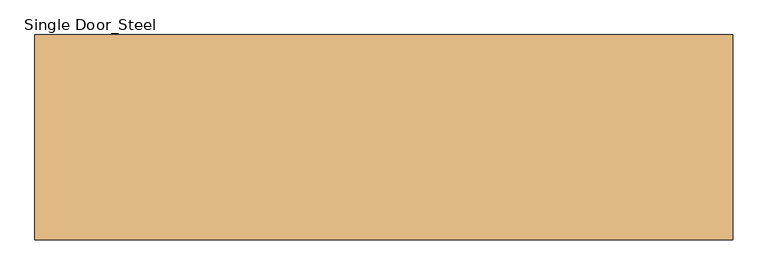
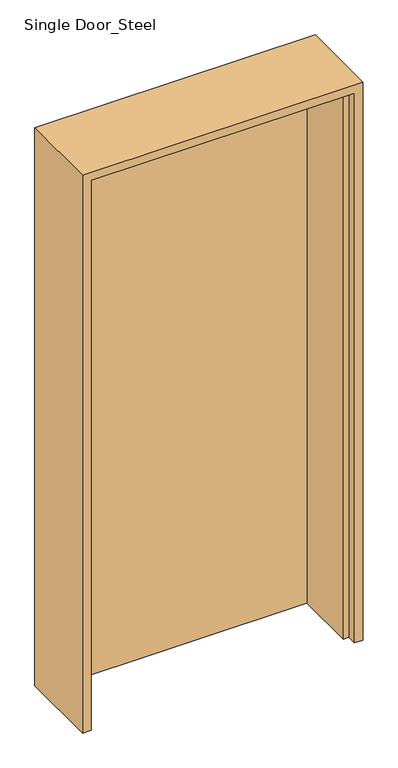
"""IFC4 building model written with IfcOpenShell, lengths in millimetres: door geometry, Single Door_Steel : H_DR_AR_B12_Single Door_Steel_W1000xH2100."""

import ifcopenshell
import ifcopenshell.guid

model = None  # the IFC model being written
_history = None  # IfcOwnerHistory: only IFC2X3 demands one
_inside = {}  # id of a spatial element -> (the spatial element, [elements in it])
_under = {}  # id of a project, library or spatial element -> (it, [spatial elements below it])
_declared = {}  # id of a project -> (the project, [libraries it declares])
_typed = {}  # id of a type object -> (the type object, [elements of that type])
_made_of = {}  # id of a material, layer set ... -> (it, [elements and type objects made of it])


def new_model(schema):
    """Start an empty IFC model of exactly this schema.

    Asked for "IFC4X3", IfcOpenShell would pick the latest addendum, in which some entities
    have other attributes; the version numbers below select the first issue.
    IFC2X3 requires an IfcOwnerHistory on every rooted entity: one is made here for all.
    """
    global model, _history
    if schema == "IFC4X3":
        model = ifcopenshell.file(schema_version=(4, 3, 0, 0))
    else:
        model = ifcopenshell.file(schema=schema)
    _inside.clear()
    _under.clear()
    _declared.clear()
    _typed.clear()
    _made_of.clear()
    _history = None
    if model.schema == "IFC2X3":
        org = make("IfcOrganization", Name="unknown")
        user = make(
            "IfcPersonAndOrganization",
            ThePerson=make("IfcPerson", FamilyName="unknown"),
            TheOrganization=org,
        )
        app = make(
            "IfcApplication",
            ApplicationDeveloper=org,
            Version="unknown",
            ApplicationFullName="unknown",
            ApplicationIdentifier="unknown",
        )
        _history = make(
            "IfcOwnerHistory",
            OwningUser=user,
            OwningApplication=app,
            ChangeAction="ADDED",
            CreationDate=0,
        )
    return model


def make(cls, **values):
    """One entity of the class cls with the attributes given. An attribute that is None is left unset."""
    return model.create_entity(
        cls, **{name: value for name, value in values.items() if value is not None}
    )


def rooted(cls, **values):
    """An entity with a GlobalId (a new one), such as an element, a storey or a relation."""
    return make(cls, GlobalId=ifcopenshell.guid.new(), OwnerHistory=_history, **values)


def si_unit(unit_type, name, prefix=None):
    """IfcSIUnit, for example si_unit("LENGTHUNIT", "METRE", prefix="MILLI")."""
    return make("IfcSIUnit", UnitType=unit_type, Prefix=prefix, Name=name)


def assignment(units):
    """IfcUnitAssignment: the units of a project."""
    return None if units is None else make("IfcUnitAssignment", Units=units)


def point(xyz):
    """IfcCartesianPoint."""
    return None if xyz is None else make("IfcCartesianPoint", Coordinates=xyz)


def direction(xyz):
    """IfcDirection."""
    return None if xyz is None else make("IfcDirection", DirectionRatios=xyz)


def frame(location, z_axis=None, x_axis=None):
    """IfcAxis2Placement3D, a coordinate frame: its origin and axes. An axis left out is left unset."""
    return make(
        "IfcAxis2Placement3D",
        Location=point(location),
        Axis=direction(z_axis),
        RefDirection=direction(x_axis),
    )


def origin():
    """The frame at (0, 0, 0) with its axes left unset."""
    return frame((0.0, 0.0, 0.0))


def origin_with_axes():
    """The frame at (0, 0, 0) with the z axis (0, 0, 1) and the x axis (1, 0, 0) written out."""
    return frame((0.0, 0.0, 0.0), z_axis=(0.0, 0.0, 1.0), x_axis=(1.0, 0.0, 0.0))


def place(relative_to, where):
    """IfcLocalPlacement: puts the frame where relative to a parent placement (None: the world)."""
    return make(
        "IfcLocalPlacement", PlacementRelTo=relative_to, RelativePlacement=where
    )


def context(
    kind, dimensions, precision=None, world=None, true_north=None, identifier=None
):
    """IfcGeometricRepresentationContext, for example the 3D "Model" context."""
    return make(
        "IfcGeometricRepresentationContext",
        ContextIdentifier=identifier,
        ContextType=kind,
        CoordinateSpaceDimension=dimensions,
        Precision=precision,
        WorldCoordinateSystem=world,
        TrueNorth=true_north,
    )


def project(units=None, contexts=None):
    """IfcProject with its units and contexts."""
    return rooted(
        "IfcProject",
        Name="project",
        RepresentationContexts=contexts,
        UnitsInContext=assignment(units),
    )


def spatial(cls, under=None, at=None, **own):
    """A site, building, storey or space (cls), placed at a placement, below another one or the project."""
    s = rooted(cls, ObjectPlacement=at, **own)
    if under is not None:
        _under.setdefault(under.id(), (under, []))[1].append(s)
    return s


def polyline(points):
    """IfcPolyline through the points."""
    return make("IfcPolyline", Points=[point(p) for p in points])


def outline(outer, holes=None, kind="AREA"):
    """IfcArbitraryClosedProfileDef: a profile drawn as a closed curve; with holes, ...WithVoids."""
    if holes is None:
        return make("IfcArbitraryClosedProfileDef", ProfileType=kind, OuterCurve=outer)
    return make(
        "IfcArbitraryProfileDefWithVoids",
        ProfileType=kind,
        OuterCurve=outer,
        InnerCurves=holes,
    )


def extrude(swept, where, along, depth):
    """IfcExtrudedAreaSolid: the profile swept, set in the frame where, extruded along a direction by depth."""
    return make(
        "IfcExtrudedAreaSolid",
        SweptArea=swept,
        Position=where,
        ExtrudedDirection=direction(along),
        Depth=depth,
    )


def faces_of(points, faces, orient=None, outer=None):
    """IfcFace entities. A face is a list of loops; a loop is a list of indices into points, from 0.

    orient and outer hold one flag for each loop. By default every Orientation is true, the
    first loop of a face is its IfcFaceOuterBound and the others are IfcFaceBound.
    """
    made = []
    for i, loops in enumerate(faces):
        bounds = []
        for j, loop in enumerate(loops):
            is_outer = j == 0 if outer is None else outer[i][j]
            bounds.append(
                make(
                    "IfcFaceOuterBound" if is_outer else "IfcFaceBound",
                    Bound=make("IfcPolyLoop", Polygon=[points[k] for k in loop]),
                    Orientation=True if orient is None else orient[i][j],
                )
            )
        made.append(make("IfcFace", Bounds=bounds))
    return made


def faceted_brep(points, faces, orient=None, outer=None, voids=None):
    """IfcFacetedBrep: a solid bounded by flat faces; with voids (closed shells), ...WithVoids."""
    shared = [point(p) for p in points]
    hull = make("IfcClosedShell", CfsFaces=faces_of(shared, faces, orient, outer))
    if voids is None:
        return make("IfcFacetedBrep", Outer=hull)
    return make(
        "IfcFacetedBrepWithVoids",
        Outer=hull,
        Voids=[
            make(cls, CfsFaces=faces_of(shared, fs, o, b)) for cls, fs, o, b in voids
        ],
    )


def shape(context_of_items, identifier, shape_type, items):
    """IfcShapeRepresentation: the items that make up one representation, for example the "Body"."""
    return make(
        "IfcShapeRepresentation",
        ContextOfItems=context_of_items,
        RepresentationIdentifier=identifier,
        RepresentationType=shape_type,
        Items=items,
    )


def source(mapping_origin, context_of_items, identifier, shape_type, items):
    """IfcRepresentationMap: a shape defined once, which mapped items show again and again."""
    return make(
        "IfcRepresentationMap",
        MappingOrigin=mapping_origin,
        MappedRepresentation=shape(context_of_items, identifier, shape_type, items),
    )


def transform(
    local_origin,
    x_axis=None,
    y_axis=None,
    z_axis=None,
    scale=None,
    scale2=None,
    scale3=None,
    uniform=True,
):
    """IfcCartesianTransformationOperator3D, or its non-uniform kind. x_axis, y_axis, z_axis: its Axis1, 2, 3."""
    if uniform:
        return make(
            "IfcCartesianTransformationOperator3D",
            Axis1=direction(x_axis),
            Axis2=direction(y_axis),
            LocalOrigin=point(local_origin),
            Scale=scale,
            Axis3=direction(z_axis),
        )
    return make(
        "IfcCartesianTransformationOperator3DnonUniform",
        Axis1=direction(x_axis),
        Axis2=direction(y_axis),
        LocalOrigin=point(local_origin),
        Scale=scale,
        Axis3=direction(z_axis),
        Scale2=scale2,
        Scale3=scale3,
    )


def mapped(mapping_source, mapping_target):
    """IfcMappedItem: shows the shape of a source again, moved by a transform."""
    return make(
        "IfcMappedItem", MappingSource=mapping_source, MappingTarget=mapping_target
    )


def made_of(thing, what):
    """Note that an element or type object is made of a material, layer set ...; save() writes the relation."""
    if what is not None:
        _made_of.setdefault(what.id(), (what, []))[1].append(thing)
    return thing


def element(
    cls,
    number,
    at=None,
    inside=None,
    cuts=None,
    type_object=None,
    material=None,
    context=None,
    identifier="Body",
    shape_type=None,
    held_by="IfcProductDefinitionShape",
    body=None,
    shapes=None,
    **own,
):
    """One element of the class cls, such as IfcWall. Its Tag is "e" and its number.

    at: its placement. inside: the storey or other place that contains it. cuts: it is an
    opening in that element (IfcRelVoidsElement). A single representation is given by context,
    identifier, shape_type and body (its items); several are given by shapes. held_by: the class
    of the entity that holds the representations. save() writes the other relations.
    """
    e = rooted(cls, Tag="e%d" % number, ObjectPlacement=at, **own)
    if body is not None:
        shapes = [shape(context, identifier, shape_type, body)]
    if shapes is not None:
        e.Representation = make(held_by, Representations=shapes)
    if inside is not None:
        _inside.setdefault(inside.id(), (inside, []))[1].append(e)
    if cuts is not None:
        rooted(
            "IfcRelVoidsElement", RelatingBuildingElement=cuts, RelatedOpeningElement=e
        )
    if type_object is not None:
        _typed.setdefault(type_object.id(), (type_object, []))[1].append(e)
    return made_of(e, material)


def aggregate(whole, parts):
    """IfcRelAggregates: a whole, such as a stair, and the parts it consists of."""
    return rooted("IfcRelAggregates", RelatingObject=whole, RelatedObjects=parts)


def save(model, path):
    """Write the relations noted so far, then the file.

    IfcRelAggregates (storeys below a building ...), IfcRelContainedInSpatialStructure (elements
    in a storey), IfcRelDefinesByType, IfcRelAssociatesMaterial and IfcRelDeclares: one each for
    every whole, place, type object, material and project.
    """
    for whole, parts in _under.values():
        aggregate(whole, parts)
    for where, things in _inside.values():
        rooted(
            "IfcRelContainedInSpatialStructure",
            RelatedElements=things,
            RelatingStructure=where,
        )
    for kind, things in _typed.values():
        rooted("IfcRelDefinesByType", RelatedObjects=things, RelatingType=kind)
    for what, things in _made_of.values():
        rooted("IfcRelAssociatesMaterial", RelatedObjects=things, RelatingMaterial=what)
    for by, libraries in _declared.values():
        rooted("IfcRelDeclares", RelatingContext=by, RelatedDefinitions=libraries)
    model.write(path)


def single_door_steel_aae97da1(model_context):
    return source(origin(), model_context, "Body", "SolidModel", [
        extrude(outline(polyline([(470.0, 147.0), (470.0, 112.0), (-470.0, 112.0), (-470.0, 147.0), (470.0, 147.0)])), origin_with_axes(), (0.0, 0.0, 1.0), 2070.0),
        faceted_brep([(470.0, 147.0, 0.0), (500.0, 147.0, 0.0), (500.0, -147.0, 0.0), (470.0, -147.0, 0.0), (470.0, -112.0, 0.0), (450.0, -112.0, 0.0), (450.0, 112.0, 0.0), (470.0, 112.0, 0.0), (470.0, 147.0, 2070.0), (-470.0, 147.0, 2070.0), (-470.0, 147.0, 0.0), (-500.0, 147.0, 0.0), (-500.0, 147.0, 2100.0), (500.0, 147.0, 2100.0), (500.0, -147.0, 2100.0), (-500.0, -147.0, 2100.0), (-500.0, -147.0, 0.0), (-470.0, -147.0, 0.0), (-470.0, -147.0, 2070.0), (470.0, -147.0, 2070.0), (470.0, -112.0, 2070.0), (-470.0, -112.0, 2070.0), (-470.0, -112.0, 0.0), (-450.0, -112.0, 0.0), (-450.0, -112.0, 2050.0), (450.0, -112.0, 2050.0), (450.0, 112.0, 2050.0), (-450.0, 112.0, 2050.0), (-450.0, 112.0, 0.0), (-470.0, 112.0, 0.0), (-470.0, 112.0, 2070.0), (470.0, 112.0, 2070.0)], [[[0, 1, 2, 3, 4, 5, 6, 7]], [[1, 0, 8, 9, 10, 11, 12, 13]], [[2, 1, 13, 14]], [[3, 2, 14, 15, 16, 17, 18, 19]], [[4, 3, 19, 20]], [[5, 4, 20, 21, 22, 23, 24, 25]], [[6, 5, 25, 26]], [[7, 6, 26, 27, 28, 29, 30, 31]], [[0, 7, 31, 8]], [[9, 30, 29, 10]], [[10, 29, 28, 23, 22, 17, 16, 11]], [[15, 12, 11, 16]], [[21, 18, 17, 22]], [[27, 24, 23, 28]], [[14, 13, 12, 15]], [[20, 19, 18, 21]], [[26, 25, 24, 27]], [[8, 31, 30, 9]]]),
    ])


if __name__ == "__main__":
    model = new_model("IFC4")
    model_context = context("Model", 3, world=origin())
    ifc_project = project(units=[si_unit("LENGTHUNIT", "METRE", prefix="MILLI")], contexts=[model_context])
    site = spatial("IfcSite", under=ifc_project)
    building = spatial("IfcBuilding", under=site)
    placement = place(None, origin())
    single_door_steel_shape = single_door_steel_aae97da1(model_context)
    element("IfcDoor", 1, ObjectType="Single Door_Steel : H_DR_AR_B12_Single Door_Steel_W1000xH2100", at=placement, inside=building, context=model_context, shape_type="MappedRepresentation", body=[
        mapped(single_door_steel_shape, transform((0.0, 0.0, 0.0), x_axis=(1.0, 0.0, 0.0), y_axis=(0.0, 1.0, 0.0), z_axis=(0.0, 0.0, 1.0))),
    ])
    save(model, "model.ifc")

# Revit data of these elements
# Type "Single Door_Steel : H_DR_AR_B12_Single Door_Steel_W1000xH2100"
#   Type Mark = "SD"
#   Analytic Construction = "<None>"
#   프레임 투영 외부. = 25 mm
#   프레임 투영 내부. = 25 mm
#   프레임 폭 = 75 mm
#   Height = 2100 mm
#   Width = 1000 mm
#   Define Thermal Properties by = 1
#   문 패널 = none
#   문 프레임 = none
#   Function = (empty or 0)
#   Wall Closure = (empty or 0)
